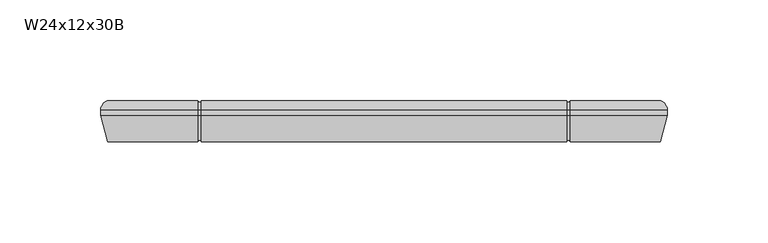
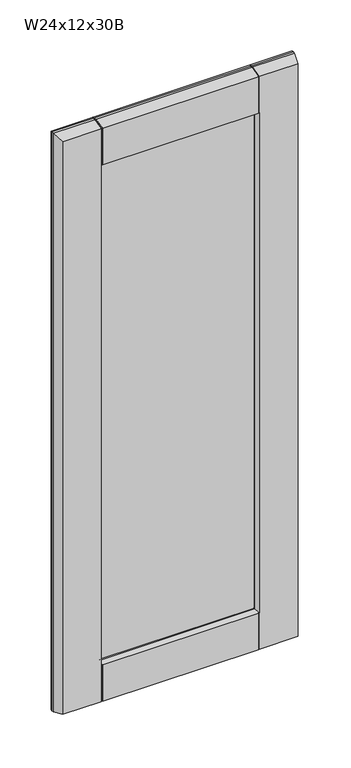
"""IFC4 building model written with IfcOpenShell, lengths in millimetres: furniture geometry, Cabinet-Wall-Merillat-Double_Door-Marlin : W24x12x30B."""

from ifc_helpers import new_model, si_unit, frame, origin, place, context, project, spatial, polyline, circle_curve, ellipse_curve, outline, extrude, source, transform, mapped, element, save
from ifc_brep_helpers import plane_surface, cylinder_surface, advanced_brep


def w24x12x30b_c7508119(model_context):
    return source(origin(), model_context, "Body", "SolidModel", [
        advanced_brep(
        [(541.0528392, 382.5621, 2108.2), (541.0528392, 382.5621, 1397.0), (537.9563467, 387.0325, 1400.0964925), (537.9563467, 387.0325, 2105.1035075), (541.0528392, 379.7935, 2108.2), (541.0528392, 379.7935, 1397.0), (537.5476392, 366.7125, 2104.6948), (537.5476392, 366.7125, 1400.5052), (492.8516765, 366.7125, 2059.9988372), (492.4815448, 367.50625, 2059.6287055), (490.4003857, 371.96931, 2057.5475465), (490.4003857, 371.96931, 1447.6524535), (492.4815448, 367.50625, 1445.5712945), (492.8516765, 366.7125, 1445.2011628), (491.8001552, 374.2094093, 2058.947316), (491.8001552, 374.2094093, 1446.252684), (506.1278392, 374.4595, 2073.275), (506.1278392, 374.4595, 1431.925), (506.1278392, 379.2855, 2073.275), (506.1278392, 379.2855, 1431.925), (491.8001552, 379.5355907, 2058.947316), (491.8001552, 379.5355907, 1446.252684), (490.4003857, 381.77569, 2057.5475465), (490.4003857, 381.77569, 1447.6524535), (492.4815448, 386.23875, 2059.6287055), (492.848809, 387.0263508, 2059.9959698), (492.8516765, 387.0325, 1445.2011628), (492.4815448, 386.23875, 1445.5712945), (263.1618317, 387.0325, 1400.0964925), (308.2295579, 387.0325, 1400.0964925), (308.2295579, 382.5621, 1397.0), (260.0653392, 382.5621, 1397.0), (492.848809, 382.5621, 1397.0), (492.848809, 387.0325, 1400.0964925), (491.261309, 382.5621, 1397.0), (309.8170579, 382.5621, 1397.0), (309.8170579, 387.0325, 1400.0964925), (491.261309, 387.0325, 1400.0964925), (308.2295579, 379.7935, 1397.0), (260.0653392, 379.7935, 1397.0), (492.848809, 379.7935, 1397.0), (491.261309, 379.7935, 1397.0), (309.8170579, 379.7935, 1397.0), (308.2295579, 366.7125, 1400.5052), (263.5705392, 366.7125, 1400.5052), (491.261309, 366.7125, 1400.5052), (309.8170579, 366.7125, 1400.5052), (492.848809, 366.7125, 1400.5052), (310.7177927, 371.96931, 1447.6524535), (308.6366337, 367.50625, 1445.5712945), (309.8170579, 367.50625, 1445.5712945), (309.8170579, 366.7125, 1445.2011628), (491.261309, 366.7125, 1445.2011628), (491.261309, 367.50625, 1445.5712945), (309.3180233, 374.2094093, 1446.252684), (294.9903392, 374.4595, 1431.925), (294.9903392, 379.2855, 1431.925), (309.3180233, 379.5355907, 1446.252684), (310.7177927, 381.77569, 1447.6524535), (491.261309, 386.23875, 1445.5712945), (491.261309, 387.0325, 1445.2011628), (309.8170579, 387.0325, 1445.2011628), (309.8170579, 386.23875, 1445.5712945), (308.6366337, 386.23875, 1445.5712945), (260.0653392, 382.5621, 2108.2), (263.1618317, 387.0325, 2105.1035075), (260.0653392, 379.7935, 2108.2), (263.5705392, 366.7125, 2104.6948), (308.266502, 366.7125, 1445.2011628), (310.7177927, 371.96931, 2057.5475465), (308.6366337, 367.50625, 2059.6287055), (308.266502, 366.7125, 2059.9988372), (309.3180233, 374.2094093, 2058.947316), (294.9903392, 374.4595, 2073.275), (294.9903392, 379.2855, 2073.275), (309.3180233, 379.5355907, 2058.947316), (310.7177927, 381.77569, 2057.5475465), (308.266502, 387.0325, 1445.2011628), (308.266502, 387.0325, 2059.9988372), (308.6366337, 386.23875, 2059.6287055), (492.848809, 387.0325, 2105.1035075), (492.848809, 382.5621, 2108.2), (308.2295579, 382.5621, 2108.2), (308.2295579, 387.0325, 2105.1035075), (309.8170579, 382.5621, 2108.2), (491.261309, 382.5621, 2108.2), (491.261309, 387.0325, 2105.1035075), (309.8170579, 387.0325, 2105.1035075), (492.848809, 379.7935, 2108.2), (308.2295579, 379.7935, 2108.2), (309.8170579, 379.7935, 2108.2), (491.261309, 379.7935, 2108.2), (492.848809, 366.7125, 2104.6948), (308.2295579, 366.7125, 2104.6948), (309.8170579, 366.7125, 2104.6948), (491.261309, 366.7125, 2104.6948), (309.8170579, 366.7125, 2059.9988372), (491.261309, 366.7125, 2059.9988372), (491.261309, 367.50625, 2059.6287055), (309.8170579, 367.50625, 2059.6287055), (309.8170579, 386.23875, 2059.6287055), (309.8170579, 387.0325, 2059.9988372), (491.261309, 387.0325, 2059.9988372), (491.261309, 386.23875, 2059.6287055), (309.8170579, 386.23875, 2104.9526052), (309.8170579, 382.5621, 2107.40625), (309.8170579, 379.8980037, 2107.40625), (309.8170579, 367.50625, 2104.0857412), (308.2295579, 367.50625, 2059.6287055), (308.2295579, 367.50625, 2104.0857412), (308.2295579, 379.8980037, 2107.40625), (308.2295579, 382.5621, 2107.40625), (308.2295579, 386.23875, 2104.9526052), (308.2295579, 386.23875, 2059.6287055), (492.848809, 386.23875, 2059.6287055), (492.848809, 386.23875, 2104.9526052), (492.848809, 382.5621, 2107.40625), (492.848809, 379.8980037, 2107.40625), (492.848809, 367.50625, 2104.0857412), (492.848809, 367.50625, 2059.6287055), (491.261309, 367.50625, 2104.0857412), (491.261309, 379.8980037, 2107.40625), (491.261309, 382.5621, 2107.40625), (491.261309, 386.23875, 2104.9526052), (492.848809, 367.50625, 1445.5712945), (492.848809, 367.50625, 1401.1142588), (492.848809, 379.8980037, 1397.79375), (492.848809, 382.5621, 1397.79375), (492.848809, 386.23875, 1400.2473948), (492.848809, 386.23875, 1445.5712945), (491.261309, 386.23875, 1400.2473948), (491.261309, 382.5621, 1397.79375), (491.261309, 379.8980037, 1397.79375), (491.261309, 367.50625, 1401.1142588), (309.8170579, 367.50625, 1401.1142588), (309.8170579, 379.8980037, 1397.79375), (309.8170579, 382.5621, 1397.79375), (309.8170579, 386.23875, 1400.2473948), (308.2295579, 386.23875, 1445.5712945), (308.2295579, 386.23875, 1400.2473948), (308.2295579, 382.5621, 1397.79375), (308.2295579, 379.8980037, 1397.79375), (308.2295579, 367.50625, 1401.1142588), (308.2295579, 367.50625, 1445.5712945)],
        [
            (0, 1),
            (1, 2, ellipse_curve(frame((536.2776392, 382.5621, 1401.7752), z_axis=(0.7071067811865475, 0.0, 0.7071067811865475), x_axis=(-0.7071067811865474, 0.0, 0.7071067811865476)), 6.7531526, 4.7752)),
            (2, 3),
            (3, 0, ellipse_curve(frame((536.2776392, 382.5621, 2103.4248), z_axis=(0.7071067811865475, 0.0, -0.7071067811865475), x_axis=(0.7071067811865474, 0.0, 0.7071067811865476)), 6.7531526, 4.7752)),
            (0, 4),
            (4, 5),
            (5, 1),
            (4, 6),
            (6, 7),
            (7, 5),
            (8, 9),
            (9, 10),
            (10, 11),
            (11, 12),
            (12, 13),
            (13, 8),
            (10, 14, ellipse_curve(frame((491.8276392, 372.6348492, 2058.9748), z_axis=(0.7071067811865475, 0.0, -0.7071067811865475), x_axis=(0.7071067811865474, 0.0, 0.7071067811865476)), 2.2271035, 1.5748)),
            (14, 15),
            (15, 11, ellipse_curve(frame((491.8276392, 372.6348492, 1446.2252), z_axis=(0.7071067811865475, 0.0, 0.7071067811865475), x_axis=(-0.7071067811865474, 0.0, 0.7071067811865476)), 2.2271035, 1.5748)),
            (14, 16),
            (16, 17),
            (17, 15),
            (16, 18),
            (18, 19),
            (19, 17),
            (18, 20),
            (20, 21),
            (21, 19),
            (20, 22, ellipse_curve(frame((491.8276392, 381.1101508, 2058.9748), z_axis=(0.7071067811865475, 0.0, -0.7071067811865475), x_axis=(0.7071067811865474, 0.0, 0.7071067811865476)), 2.2271035, 1.5748)),
            (22, 23),
            (23, 21, ellipse_curve(frame((491.8276392, 381.1101508, 1446.2252), z_axis=(0.7071067811865475, 0.0, 0.7071067811865475), x_axis=(-0.7071067811865474, 0.0, 0.7071067811865476)), 2.2271035, 1.5748)),
            (22, 24),
            (24, 25),
            (25, 26),
            (26, 27),
            (27, 23),
            (28, 29),
            (29, 30, circle_curve(frame((308.2295579, 382.5621, 1401.7752), z_axis=(-1.0, 0.0, 0.0), x_axis=(0.0, -1.0, 0.0)), 4.7752)),
            (30, 31),
            (31, 28, ellipse_curve(frame((264.8405392, 382.5621, 1401.7752), z_axis=(0.7071067811865475, 0.0, -0.7071067811865475), x_axis=(0.7071067811865476, 0.0, 0.7071067811865474)), 6.7531526, 4.7752)),
            (1, 32),
            (32, 33, circle_curve(frame((492.848809, 382.5621, 1401.7752), z_axis=(1.0, 0.0, 0.0), x_axis=(0.0, -1.0, 0.0)), 4.7752)),
            (33, 2),
            (34, 35),
            (35, 36, circle_curve(frame((309.8170579, 382.5621, 1401.7752), z_axis=(1.0, 0.0, 0.0), x_axis=(0.0, -1.0, 0.0)), 4.7752)),
            (36, 37),
            (37, 34, circle_curve(frame((491.261309, 382.5621, 1401.7752), z_axis=(-1.0, 0.0, 0.0), x_axis=(0.0, -1.0, 0.0)), 4.7752)),
            (30, 38),
            (38, 39),
            (39, 31),
            (5, 40),
            (40, 32),
            (41, 42),
            (42, 35),
            (34, 41),
            (38, 43),
            (43, 44),
            (44, 39),
            (45, 46),
            (46, 42),
            (41, 45),
            (7, 47),
            (47, 40),
            (48, 49),
            (49, 50),
            (50, 51),
            (51, 52),
            (52, 53),
            (53, 12),
            (11, 48),
            (15, 54),
            (54, 48, ellipse_curve(frame((309.2905392, 372.6348492, 1446.2252), z_axis=(0.7071067811865475, 0.0, -0.7071067811865475), x_axis=(0.7071067811865476, 0.0, 0.7071067811865474)), 2.2271035, 1.5748)),
            (17, 55),
            (55, 54),
            (19, 56),
            (56, 55),
            (21, 57),
            (57, 56),
            (23, 58),
            (58, 57, ellipse_curve(frame((309.2905392, 381.1101508, 1446.2252), z_axis=(0.7071067811865475, 0.0, -0.7071067811865475), x_axis=(0.7071067811865476, 0.0, 0.7071067811865474)), 2.2271035, 1.5748)),
            (27, 59),
            (59, 60),
            (60, 61),
            (61, 62),
            (62, 63),
            (63, 58),
            (31, 64),
            (64, 65, ellipse_curve(frame((264.8405392, 382.5621, 2103.4248), z_axis=(-0.7071067811865475, 0.0, -0.7071067811865475), x_axis=(0.7071067811865474, 0.0, -0.7071067811865476)), 6.7531526, 4.7752)),
            (65, 28),
            (39, 66),
            (66, 64),
            (44, 67),
            (67, 66),
            (68, 49),
            (48, 69),
            (69, 70),
            (70, 71),
            (71, 68),
            (54, 72),
            (72, 69, ellipse_curve(frame((309.2905392, 372.6348492, 2058.9748), z_axis=(-0.7071067811865475, 0.0, -0.7071067811865475), x_axis=(0.7071067811865474, 0.0, -0.7071067811865476)), 2.2271035, 1.5748)),
            (55, 73),
            (73, 72),
            (56, 74),
            (74, 73),
            (57, 75),
            (75, 74),
            (58, 76),
            (76, 75, ellipse_curve(frame((309.2905392, 381.1101508, 2058.9748), z_axis=(-0.7071067811865475, 0.0, -0.7071067811865475), x_axis=(0.7071067811865474, 0.0, -0.7071067811865476)), 2.2271035, 1.5748)),
            (63, 77),
            (77, 78),
            (78, 79),
            (79, 76),
            (3, 80),
            (80, 81, circle_curve(frame((492.848809, 382.5621, 2103.4248), z_axis=(1.0, 0.0, 0.0), x_axis=(0.0, -1.0, 0.0)), 4.7752)),
            (81, 0),
            (64, 82),
            (82, 83, circle_curve(frame((308.2295579, 382.5621, 2103.4248), z_axis=(-1.0, 0.0, 0.0), x_axis=(0.0, -1.0, 0.0)), 4.7752)),
            (83, 65),
            (84, 85),
            (85, 86, circle_curve(frame((491.261309, 382.5621, 2103.4248), z_axis=(-1.0, 0.0, 0.0), x_axis=(0.0, -1.0, 0.0)), 4.7752)),
            (86, 87),
            (87, 84, circle_curve(frame((309.8170579, 382.5621, 2103.4248), z_axis=(1.0, 0.0, 0.0), x_axis=(0.0, -1.0, 0.0)), 4.7752)),
            (81, 88),
            (88, 4),
            (66, 89),
            (89, 82),
            (90, 91),
            (91, 85),
            (84, 90),
            (88, 92),
            (92, 6),
            (67, 93),
            (93, 89),
            (94, 95),
            (95, 91),
            (90, 94),
            (51, 46),
            (45, 52),
            (43, 68),
            (71, 93),
            (92, 8),
            (13, 47),
            (96, 97),
            (97, 95),
            (94, 96),
            (9, 98),
            (98, 97),
            (96, 99),
            (99, 70),
            (69, 10),
            (72, 14),
            (73, 16),
            (74, 18),
            (75, 20),
            (76, 22),
            (79, 100),
            (100, 101),
            (101, 102),
            (102, 103),
            (103, 24),
            (33, 26),
            (25, 80),
            (36, 61),
            (60, 37),
            (83, 78),
            (77, 29),
            (86, 102),
            (101, 87),
            (100, 104),
            (104, 105, circle_curve(frame((309.8170579, 382.5621, 2103.4248), z_axis=(1.0, 0.0, 0.0), x_axis=(0.0, 0.0, 1.0)), 3.98145)),
            (105, 106),
            (106, 107),
            (107, 99),
            (71, 108),
            (108, 109),
            (109, 110),
            (110, 111),
            (111, 112, circle_curve(frame((308.2295579, 382.5621, 2103.4248), z_axis=(-1.0, 0.0, 0.0), x_axis=(0.0, 0.0, 1.0)), 3.98145)),
            (112, 113),
            (113, 78),
            (113, 79),
            (112, 104),
            (111, 105),
            (110, 106),
            (109, 107),
            (108, 70),
            (25, 114),
            (114, 115),
            (115, 116, circle_curve(frame((492.848809, 382.5621, 2103.4248), z_axis=(1.0, 0.0, 0.0), x_axis=(0.0, 0.0, 1.0)), 3.98145)),
            (116, 117),
            (117, 118),
            (118, 119),
            (119, 8),
            (98, 120),
            (120, 121),
            (121, 122),
            (122, 123, circle_curve(frame((491.261309, 382.5621, 2103.4248), z_axis=(-1.0, 0.0, 0.0), x_axis=(0.0, 0.0, 1.0)), 3.98145)),
            (123, 103),
            (24, 114),
            (123, 115),
            (122, 116),
            (121, 117),
            (120, 118),
            (9, 119),
            (13, 124),
            (124, 125),
            (125, 126),
            (126, 127),
            (127, 128, circle_curve(frame((492.848809, 382.5621, 1401.7752), z_axis=(1.0, 0.0, 0.0), x_axis=(0.0, 0.0, 1.0)), 3.98145)),
            (128, 129),
            (129, 26),
            (59, 130),
            (130, 131, circle_curve(frame((491.261309, 382.5621, 1401.7752), z_axis=(-1.0, 0.0, 0.0), x_axis=(0.0, 0.0, 1.0)), 3.98145)),
            (131, 132),
            (132, 133),
            (133, 53),
            (12, 124),
            (133, 125),
            (132, 126),
            (131, 127),
            (130, 128),
            (27, 129),
            (50, 134),
            (134, 135),
            (135, 136),
            (136, 137, circle_curve(frame((309.8170579, 382.5621, 1401.7752), z_axis=(1.0, 0.0, 0.0), x_axis=(0.0, 0.0, 1.0)), 3.98145)),
            (137, 62),
            (138, 139),
            (139, 140, circle_curve(frame((308.2295579, 382.5621, 1401.7752), z_axis=(-1.0, 0.0, 0.0), x_axis=(0.0, 0.0, 1.0)), 3.98145)),
            (140, 141),
            (141, 142),
            (142, 143),
            (143, 68),
            (77, 138),
            (63, 138),
            (143, 49),
            (142, 134),
            (141, 135),
            (140, 136),
            (139, 137),
        ],
        [
            cylinder_surface(frame((536.2776392, 382.5621, 2108.2), z_axis=(0.0, 0.0, 1.0), x_axis=(0.0, -1.0, 0.0)), 4.7752),
            plane_surface(frame((541.0528392, 382.5621, 2108.2), z_axis=(1.0, 0.0, 0.0), x_axis=(0.0, 0.0, -1.0))),
            plane_surface(frame((541.0528392, 379.7935, 2108.2), z_axis=(0.9659229350723619, -0.25882983502910506, 0.0), x_axis=(0.0, 0.0, -1.0))),
            plane_surface(frame((492.8516765, 366.7125, 2059.9988372), z_axis=(-0.9063077870366099, -0.4226182617407856, 0.0), x_axis=(0.0, 0.0, -1.0))),
            cylinder_surface(frame((491.8276392, 372.6348492, 2108.2), z_axis=(0.0, 0.0, 1.0000000000000002), x_axis=(-0.01745240643729364, 0.9998476951563912, 0.0)), 1.5748),
            plane_surface(frame((491.8001552, 374.2094093, 2058.947316), z_axis=(-0.017452406437322144, 0.9998476951563906, 0.0), x_axis=(0.0, 0.0, -1.0))),
            plane_surface(frame((506.1278392, 374.4595, 2073.275), z_axis=(-1.0, 0.0, 0.0), x_axis=(0.0, 0.0, -1.0))),
            plane_surface(frame((506.1278392, 379.2855, 2073.275), z_axis=(-0.01745240643727848, -0.9998476951563914, 0.0), x_axis=(0.0, 0.0, -1.0))),
            cylinder_surface(frame((491.8276392, 381.1101508, 2108.2), z_axis=(0.0, 0.0, 1.0000000000000002), x_axis=(-0.9063077870367326, 0.42261826174052236, 0.0)), 1.5748),
            plane_surface(frame((490.4003857, 381.77569, 2057.5475465), z_axis=(-0.9063077870366333, 0.4226182617407352, 0.0), x_axis=(0.0, 0.0, -1.0))),
            cylinder_surface(frame((541.0528392, 382.5621, 1401.7752), z_axis=(1.0, 0.0, 0.0), x_axis=(0.0, -1.0, 0.0)), 4.7752),
            plane_surface(frame((541.0528392, 382.5621, 1397.0), z_axis=(0.0, 0.0, -1.0), x_axis=(-1.0, 0.0, 0.0))),
            plane_surface(frame((541.0528392, 379.7935, 1397.0), z_axis=(0.0, -0.2588298350291095, -0.9659229350723607), x_axis=(-1.0, 0.0, 0.0))),
            plane_surface(frame((492.8516765, 366.7125, 1445.2011628), z_axis=(0.0, -0.42261826174078143, 0.9063077870366119), x_axis=(-1.0, 0.0, 0.0))),
            cylinder_surface(frame((541.0528392, 372.6348492, 1446.2252), z_axis=(1.0000000000000002, 0.0, 0.0), x_axis=(0.0, 0.9998476951563913, 0.017452406437289025)), 1.5748),
            plane_surface(frame((491.8001552, 374.2094093, 1446.252684), z_axis=(0.0, 0.9998476951563907, 0.01745240643731753), x_axis=(-1.0, 0.0, 0.0))),
            plane_surface(frame((506.1278392, 374.4595, 1431.925), z_axis=(0.0, 0.0, 1.0), x_axis=(-1.0, 0.0, 0.0))),
            plane_surface(frame((506.1278392, 379.2855, 1431.925), z_axis=(0.0, -0.9998476951563913, 0.017452406437283095), x_axis=(-1.0, 0.0, 0.0))),
            cylinder_surface(frame((541.0528392, 381.1101508, 1446.2252), z_axis=(1.0000000000000002, 0.0, 0.0), x_axis=(0.0, 0.4226182617405265, 0.9063077870367306)), 1.5748),
            plane_surface(frame((490.4003857, 381.77569, 1447.6524535), z_axis=(0.0, 0.4226182617407394, 0.9063077870366314), x_axis=(-1.0, 0.0, 0.0))),
            cylinder_surface(frame((264.8405392, 382.5621, 1397.0), z_axis=(0.0, 0.0, -1.0), x_axis=(0.0, -1.0, 0.0)), 4.7752),
            plane_surface(frame((260.0653392, 382.5621, 1397.0), z_axis=(-1.0, 0.0, 0.0), x_axis=(0.0, 0.0, 1.0))),
            plane_surface(frame((260.0653392, 379.7935, 1397.0), z_axis=(-0.9659229350723619, -0.25882983502910506, 0.0), x_axis=(0.0, 0.0, 1.0))),
            plane_surface(frame((308.266502, 366.7125, 1445.2011628), z_axis=(0.9063077870366099, -0.4226182617407856, 0.0), x_axis=(0.0, 0.0, 1.0))),
            cylinder_surface(frame((309.2905392, 372.6348492, 1397.0), z_axis=(0.0, 0.0, -1.0000000000000002), x_axis=(0.01745240643729364, 0.9998476951563912, 0.0)), 1.5748),
            plane_surface(frame((309.3180233, 374.2094093, 1446.252684), z_axis=(0.017452406437322144, 0.9998476951563906, 0.0), x_axis=(0.0, 0.0, 1.0))),
            plane_surface(frame((294.9903392, 374.4595, 1431.925), z_axis=(1.0, 0.0, 0.0), x_axis=(0.0, 0.0, 1.0))),
            plane_surface(frame((294.9903392, 379.2855, 1431.925), z_axis=(0.01745240643727848, -0.9998476951563914, 0.0), x_axis=(0.0, 0.0, 1.0))),
            cylinder_surface(frame((309.2905392, 381.1101508, 1397.0), z_axis=(0.0, 0.0, -1.0000000000000002), x_axis=(0.9063077870367326, 0.42261826174052236, 0.0)), 1.5748),
            plane_surface(frame((310.7177927, 381.77569, 1447.6524535), z_axis=(0.9063077870366333, 0.4226182617407352, 0.0), x_axis=(0.0, 0.0, 1.0))),
            cylinder_surface(frame((260.0653392, 382.5621, 2103.4248), z_axis=(-1.0, 0.0, 0.0), x_axis=(0.0, -1.0, 0.0)), 4.7752),
            plane_surface(frame((260.0653392, 382.5621, 2108.2), z_axis=(0.0, 0.0, 1.0), x_axis=(1.0, 0.0, 0.0))),
            plane_surface(frame((260.0653392, 379.7935, 2108.2), z_axis=(0.0, -0.2588298350291006, 0.9659229350723632), x_axis=(1.0, 0.0, 0.0))),
            plane_surface(frame((263.5705392, 366.7125, 2104.6948), z_axis=(0.0, -1.0, 0.0), x_axis=(1.0, 0.0, 0.0))),
            plane_surface(frame((308.266502, 366.7125, 2059.9988372), z_axis=(0.0, -0.42261826174078976, -0.9063077870366079), x_axis=(1.0, 0.0, 0.0))),
            cylinder_surface(frame((260.0653392, 372.6348492, 2058.9748), z_axis=(-1.0000000000000002, 0.0, 0.0), x_axis=(0.0, 0.999847695156391, -0.017452406437298253)), 1.5748),
            plane_surface(frame((309.3180233, 374.2094093, 2058.947316), z_axis=(0.0, 0.9998476951563905, -0.01745240643732676), x_axis=(1.0, 0.0, 0.0))),
            plane_surface(frame((294.9903392, 374.4595, 2073.275), z_axis=(0.0, 0.0, -1.0), x_axis=(1.0, 0.0, 0.0))),
            plane_surface(frame((294.9903392, 379.2855, 2073.275), z_axis=(0.0, -0.9998476951563915, -0.017452406437273867), x_axis=(1.0, 0.0, 0.0))),
            cylinder_surface(frame((260.0653392, 381.1101508, 2058.9748), z_axis=(-1.0000000000000002, 0.0, 0.0), x_axis=(0.0, 0.4226182617405182, -0.9063077870367346)), 1.5748),
            plane_surface(frame((310.7177927, 381.77569, 2057.5475465), z_axis=(0.0, 0.422618261740731, -0.9063077870366353), x_axis=(1.0, 0.0, 0.0))),
            plane_surface(frame((308.266502, 387.0325, 2059.9988372), z_axis=(0.0, 1.0, 0.0), x_axis=(1.0, 0.0, 0.0))),
            plane_surface(frame((309.8170579, 387.0325, 2059.9988372), z_axis=(-1.0000000000000002, 0.0, 0.0), x_axis=(0.0, -0.9063077870366335, -0.422618261740735))),
            plane_surface(frame((308.2295579, 387.0325, 2059.9988372), z_axis=(1.0000000000000002, 0.0, 0.0), x_axis=(0.0, 0.9063077870366335, 0.422618261740735))),
            plane_surface(frame((309.8170579, 387.0325, 2059.9988372), z_axis=(0.0, -0.422618261740735, 0.9063077870366335), x_axis=(-1.0, 0.0, 0.0))),
            plane_surface(frame((309.8170579, 386.23875, 2059.6287055), z_axis=(0.0, 1.0, 0.0), x_axis=(-1.0, 0.0, 0.0))),
            cylinder_surface(frame((308.2295579, 382.5621, 2103.4248), z_axis=(-1.0, 0.0, 0.0), x_axis=(0.0, 0.0, 1.0)), 3.98145),
            plane_surface(frame((309.8170579, 382.5621, 2107.40625), z_axis=(0.0, 0.0, 1.0), x_axis=(-1.0, 0.0, 0.0))),
            plane_surface(frame((309.8170579, 379.8980037, 2107.40625), z_axis=(0.0, -0.2588298350291711, 0.9659229350723443), x_axis=(-1.0, 0.0, 0.0))),
            plane_surface(frame((309.8170579, 367.50625, 2104.0857412), z_axis=(0.0, -1.0, 0.0), x_axis=(-1.0, 0.0, 0.0))),
            plane_surface(frame((309.8170579, 367.50625, 2059.6287055), z_axis=(0.0, 0.4226182617408151, 0.906307787036596), x_axis=(-1.0, 0.0, 0.0))),
            plane_surface(frame((492.848809, 387.0325, 2059.9988372), z_axis=(-1.0000000000000002, 0.0, 0.0), x_axis=(0.0, -0.9063077870366413, -0.42261826174071837))),
            plane_surface(frame((491.261309, 387.0325, 2059.9988372), z_axis=(1.0000000000000002, 0.0, 0.0), x_axis=(0.0, 0.9063077870366413, 0.42261826174071837))),
            plane_surface(frame((492.848809, 387.0325, 2059.9988372), z_axis=(0.0, -0.42261826174071837, 0.9063077870366413), x_axis=(-1.0, 0.0, 0.0))),
            plane_surface(frame((492.848809, 386.23875, 2059.6287055), z_axis=(0.0, 1.0, 0.0), x_axis=(-1.0, 0.0, 0.0))),
            cylinder_surface(frame((491.261309, 382.5621, 2103.4248), z_axis=(-1.0, 0.0, 0.0), x_axis=(0.0, 0.0, 1.0)), 3.98145),
            plane_surface(frame((492.848809, 382.5621, 2107.40625), z_axis=(0.0, 0.0, 1.0), x_axis=(-1.0, 0.0, 0.0))),
            plane_surface(frame((492.848809, 379.8980037, 2107.40625), z_axis=(0.0, -0.2588298350291734, 0.9659229350723437), x_axis=(-1.0, 0.0, 0.0))),
            plane_surface(frame((492.848809, 367.50625, 2104.0857412), z_axis=(0.0, -1.0, 0.0), x_axis=(-1.0, 0.0, 0.0))),
            plane_surface(frame((492.848809, 367.50625, 2059.6287055), z_axis=(0.0, 0.4226182617408322, 0.9063077870365881), x_axis=(-1.0, 0.0, 0.0))),
            plane_surface(frame((492.848809, 382.5621, 1406.5504), z_axis=(-1.0, 0.0, 0.0), x_axis=(0.0, 1.0, 0.0))),
            plane_surface(frame((491.261309, 382.5621, 1406.5504), z_axis=(1.0, 0.0, 0.0), x_axis=(0.0, -1.0, 0.0))),
            plane_surface(frame((492.848809, 366.7125, 1445.2011628), z_axis=(0.0, 0.4226182617408193, -0.906307787036594), x_axis=(-1.0, 0.0, 0.0))),
            plane_surface(frame((492.848809, 367.50625, 1445.5712945), z_axis=(0.0, -1.0, 0.0), x_axis=(-1.0, 0.0, 0.0))),
            plane_surface(frame((492.848809, 367.50625, 1401.1142588), z_axis=(0.0, -0.258829835029436, -0.9659229350722732), x_axis=(-1.0, 0.0, 0.0))),
            plane_surface(frame((492.848809, 379.8980037, 1397.79375), z_axis=(0.0, 0.0, -1.0), x_axis=(-1.0, 0.0, 0.0))),
            cylinder_surface(frame((491.261309, 382.5621, 1401.7752), z_axis=(-1.0, 0.0, 0.0), x_axis=(0.0, 0.0, 1.0)), 3.98145),
            plane_surface(frame((492.848809, 386.23875, 1400.2473948), z_axis=(0.0, 1.0, 0.0), x_axis=(-1.0, 0.0, 0.0))),
            plane_surface(frame((492.848809, 386.23875, 1445.5712945), z_axis=(0.0, -0.42261826174073513, -0.9063077870366334), x_axis=(-1.0, 0.0, 0.0))),
            plane_surface(frame((309.8170579, 386.23875, 1445.5712945), z_axis=(-1.0, 0.0, 0.0), x_axis=(0.0, 0.9063077870366235, -0.4226182617407563))),
            plane_surface(frame((308.2295579, 386.23875, 1445.5712945), z_axis=(1.0, 0.0, 0.0), x_axis=(0.0, -0.9063077870366235, 0.4226182617407563))),
            plane_surface(frame((309.8170579, 386.23875, 1445.5712945), z_axis=(0.0, -0.4226182617407563, -0.9063077870366235), x_axis=(-1.0, 0.0, 0.0))),
            plane_surface(frame((309.8170579, 366.7125, 1445.2011628), z_axis=(0.0, 0.42261826174079387, -0.9063077870366061), x_axis=(-1.0, 0.0, 0.0))),
            plane_surface(frame((309.8170579, 367.50625, 1445.5712945), z_axis=(0.0, -1.0, 0.0), x_axis=(-1.0, 0.0, 0.0))),
            plane_surface(frame((309.8170579, 367.50625, 1401.1142588), z_axis=(0.0, -0.258829835029439, -0.9659229350722724), x_axis=(-1.0, 0.0, 0.0))),
            plane_surface(frame((309.8170579, 379.8980037, 1397.79375), z_axis=(0.0, 0.0, -1.0), x_axis=(-1.0, 0.0, 0.0))),
            cylinder_surface(frame((308.2295579, 382.5621, 1401.7752), z_axis=(-1.0, 0.0, 0.0), x_axis=(0.0, 0.0, 1.0)), 3.98145),
            plane_surface(frame((309.8170579, 386.23875, 1400.2473948), z_axis=(0.0, 1.0, 0.0), x_axis=(-1.0, 0.0, 0.0))),
        ],
        [
            (0, [[1, 2, 3, 4]]),
            (1, [[5, 6, 7, -1]]),
            (2, [[8, 9, 10, -6]]),
            (3, [[11, 12, 13, 14, 15, 16]]),
            (4, [[17, 18, 19, -13]]),
            (5, [[20, 21, 22, -18]]),
            (6, [[23, 24, 25, -21]]),
            (7, [[26, 27, 28, -24]]),
            (8, [[29, 30, 31, -27]]),
            (9, [[32, 33, 34, 35, 36, -30]]),
            (10, [[37, 38, 39, 40]]),
            (10, [[41, 42, 43, -2]]),
            (10, [[44, 45, 46, 47]]),
            (11, [[-39, 48, 49, 50]]),
            (11, [[51, 52, -41, -7]]),
            (11, [[53, 54, -44, 55]]),
            (12, [[-49, 56, 57, 58]]),
            (12, [[59, 60, -53, 61]]),
            (12, [[62, 63, -51, -10]]),
            (13, [[64, 65, 66, 67, 68, 69, -14, 70]]),
            (14, [[71, 72, -70, -19]]),
            (15, [[73, 74, -71, -22]]),
            (16, [[75, 76, -73, -25]]),
            (17, [[77, 78, -75, -28]]),
            (18, [[79, 80, -77, -31]]),
            (19, [[-36, 81, 82, 83, 84, 85, 86, -79]]),
            (20, [[87, 88, 89, -40]]),
            (21, [[90, 91, -87, -50]]),
            (22, [[92, 93, -90, -58]]),
            (23, [[94, -64, 95, 96, 97, 98]]),
            (24, [[99, 100, -95, -72]]),
            (25, [[101, 102, -99, -74]]),
            (26, [[103, 104, -101, -76]]),
            (27, [[105, 106, -103, -78]]),
            (28, [[107, 108, -105, -80]]),
            (29, [[-86, 109, 110, 111, 112, -107]]),
            (30, [[113, 114, 115, -4]]),
            (30, [[116, 117, 118, -88]]),
            (30, [[119, 120, 121, 122]]),
            (31, [[-115, 123, 124, -5]]),
            (31, [[125, 126, -116, -91]]),
            (31, [[127, 128, -119, 129]]),
            (32, [[-124, 130, 131, -8]]),
            (32, [[132, 133, -125, -93]]),
            (32, [[134, 135, -127, 136]]),
            (33, [[-67, 137, -59, 138]]),
            (33, [[-57, 139, -98, 140, -132, -92]]),
            (33, [[-131, 141, -16, 142, -62, -9]]),
            (33, [[143, 144, -134, 145]]),
            (34, [[-12, 146, 147, -143, 148, 149, -96, 150]]),
            (35, [[-150, -100, 151, -17]]),
            (36, [[-151, -102, 152, -20]]),
            (37, [[-152, -104, 153, -23]]),
            (38, [[-153, -106, 154, -26]]),
            (39, [[-154, -108, 155, -29]]),
            (40, [[-112, 156, 157, 158, 159, 160, -32, -155]]),
            (41, [[-43, 161, -34, 162, -113, -3]]),
            (41, [[-46, 163, -83, 164]]),
            (41, [[-118, 165, -110, 166, -37, -89]]),
            (41, [[-121, 167, -158, 168]]),
            (42, [[-148, -145, -136, -129, -122, -168, -157, 169, 170, 171, 172, 173]]),
            (43, [[-165, -117, -126, -133, -140, 174, 175, 176, 177, 178, 179, 180]]),
            (44, [[181, -111, -180]]),
            (45, [[-156, -181, -179, 182, -169]]),
            (46, [[-182, -178, 183, -170]]),
            (47, [[-183, -177, 184, -171]]),
            (48, [[-184, -176, 185, -172]]),
            (49, [[-185, -175, 186, -149, -173]]),
            (50, [[-97, -186, -174]]),
            (51, [[-141, -130, -123, -114, -162, 187, 188, 189, 190, 191, 192, 193]]),
            (52, [[-159, -167, -120, -128, -135, -144, -147, 194, 195, 196, 197, 198]]),
            (53, [[-33, 199, -187]]),
            (54, [[-199, -160, -198, 200, -188]]),
            (55, [[-200, -197, 201, -189]]),
            (56, [[-201, -196, 202, -190]]),
            (57, [[-202, -195, 203, -191]]),
            (58, [[-203, -194, -146, 204, -192]]),
            (59, [[-204, -11, -193]]),
            (60, [[-161, -42, -52, -63, -142, 205, 206, 207, 208, 209, 210, 211]]),
            (61, [[-68, -138, -61, -55, -47, -164, -82, 212, 213, 214, 215, 216]]),
            (62, [[-15, 217, -205]]),
            (63, [[-217, -69, -216, 218, -206]]),
            (64, [[-218, -215, 219, -207]]),
            (65, [[-219, -214, 220, -208]]),
            (66, [[-220, -213, 221, -209]]),
            (67, [[-221, -212, -81, 222, -210]]),
            (68, [[-222, -35, -211]]),
            (69, [[-84, -163, -45, -54, -60, -137, -66, 223, 224, 225, 226, 227]]),
            (70, [[228, 229, 230, 231, 232, 233, -139, -56, -48, -38, -166, 234]]),
            (71, [[-109, 235, -234]]),
            (72, [[236, -94, -233]]),
            (73, [[-65, -236, -232, 237, -223]]),
            (74, [[-237, -231, 238, -224]]),
            (75, [[-238, -230, 239, -225]]),
            (76, [[-239, -229, 240, -226]]),
            (77, [[-240, -228, -235, -85, -227]]),
        ],
    ),
        extrude(outline(polyline([(294.9903392, 379.2855), (506.1278392, 379.2855), (506.1278392, 374.4595), (294.9903392, 374.4595), (294.9903392, 379.2855)])), frame((0.0, 0.0, 1431.925), z_axis=(0.0, 0.0, 1.0), x_axis=(1.0, 0.0, 0.0)), (0.0, 0.0, 1.0), 641.35),
    ])


if __name__ == "__main__":
    model = new_model("IFC4")
    model_context = context("Model", 3, world=origin())
    ifc_project = project(units=[si_unit("LENGTHUNIT", "METRE", prefix="MILLI")], contexts=[model_context])
    site = spatial("IfcSite", under=ifc_project)
    building = spatial("IfcBuilding", under=site)
    placement = place(None, origin())
    w24x12x30b_shape = w24x12x30b_c7508119(model_context)
    element("IfcFurniture", 1, ObjectType="Cabinet-Wall-Merillat-Double_Door-Marlin : W24x12x30B", at=placement, inside=building, context=model_context, shape_type="MappedRepresentation", body=[
        mapped(w24x12x30b_shape, transform((0.0, 0.0, 0.0), x_axis=(1.0, 0.0, 0.0), y_axis=(0.0, 1.0, 0.0), z_axis=(0.0, 0.0, 1.0))),
    ])
    save(model, "model.ifc")

# Revit data of these elements
# Type "Cabinet-Wall-Merillat-Double_Door-Marlin : W24x12x30B"
#   URL = "https://www.merillat.com/"
#   Product Page URL = "https://www.merillat.com/our-products/"
#   Product Line = "Express"
#   Product Group = "Wall Cabinet"
#   Product Documentation Link = "http://merillatbusiness.com/wp-content/uploads/2014/07/Merillat_Classic_Catalog.pdf"
#   Model = "W2442B"
#   Manufacturer = "Merillat"
#   Height Note = "Actual Height of 21 inches Cabinet is 20 1/2 inches"
#   Glass Door Note = "Glass Cabinet doors are only available in specific sizes. Please refer to the catalog for this information before requesting a glass size."
#   Finish = "Wood"
#   Description = "Wall 2442 Butt Door"
#   Construction Type = "Wall Cabinet"
#   Cabinet Construction Note = "Cabinets with B suffix have BUTT doors without a center frame stile:"
#   Assembly Code = "C1030410"
#   Spacing = 0' - 1"
#   Shelving Height = 0' - 6 3/4"
#   Door Spacing = 0' - 0 1/8"
#   Cabinet Door Width = 0' - 11 1/16"
#   Cabinet Door Height = 2' - 4"
#   Depth = 1' - 0"
#   Height = 2' - 6"
#   Top Of Cabinet = 7' - 0"
#   Width = 2' - 0"
#   COBie.Type = no
#   Top and Bottom Visibility = yes
#   Partial Overlay Butt = yes
#   Partial Overlay = no
#   Number of Shelves Greater than one = 3
#   Number of Shelves = 3
#   Middle Shelf = yes
#   Full Overlay Butt = no
#   Full Overlay = no
#   Elevation Swing Line = yes
#   Door Drawer Material = Wood - Merillat - Pecan(1)
#   Cabinet Material = Wood - Merillat - Pecan(1)
#   Cabinet Door Style = element 806847
# Element 1 (IfcFurniture, "Cabinet-Wall-Merillat-Double_Door-Marlin : W24x12x30B")
#   Materials on its faces: "Wood - Merillat - Pecan(1)"
# Materials
#   "Wood - Merillat - Pecan(1)": class "Wood", colour RGB 108 67 43, transparency 0, Cost = 0
